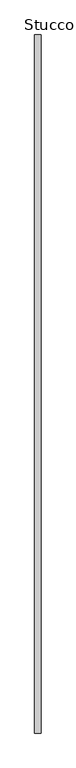
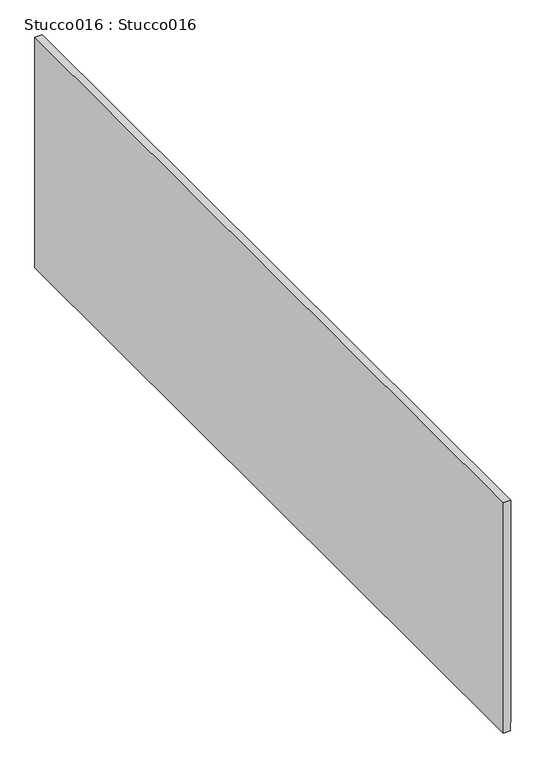
"""IFC4 building model written with IfcOpenShell, lengths in millimetres: proxy geometry, Stucco016 : Stucco016."""

import ifcopenshell
import ifcopenshell.guid

model = None  # the IFC model being written
_history = None  # IfcOwnerHistory: only IFC2X3 demands one
_inside = {}  # id of a spatial element -> (the spatial element, [elements in it])
_under = {}  # id of a project, library or spatial element -> (it, [spatial elements below it])
_declared = {}  # id of a project -> (the project, [libraries it declares])
_typed = {}  # id of a type object -> (the type object, [elements of that type])
_made_of = {}  # id of a material, layer set ... -> (it, [elements and type objects made of it])


def new_model(schema):
    """Start an empty IFC model of exactly this schema.

    Asked for "IFC4X3", IfcOpenShell would pick the latest addendum, in which some entities
    have other attributes; the version numbers below select the first issue.
    IFC2X3 requires an IfcOwnerHistory on every rooted entity: one is made here for all.
    """
    global model, _history
    if schema == "IFC4X3":
        model = ifcopenshell.file(schema_version=(4, 3, 0, 0))
    else:
        model = ifcopenshell.file(schema=schema)
    _inside.clear()
    _under.clear()
    _declared.clear()
    _typed.clear()
    _made_of.clear()
    _history = None
    if model.schema == "IFC2X3":
        org = make("IfcOrganization", Name="unknown")
        user = make(
            "IfcPersonAndOrganization",
            ThePerson=make("IfcPerson", FamilyName="unknown"),
            TheOrganization=org,
        )
        app = make(
            "IfcApplication",
            ApplicationDeveloper=org,
            Version="unknown",
            ApplicationFullName="unknown",
            ApplicationIdentifier="unknown",
        )
        _history = make(
            "IfcOwnerHistory",
            OwningUser=user,
            OwningApplication=app,
            ChangeAction="ADDED",
            CreationDate=0,
        )
    return model


def make(cls, **values):
    """One entity of the class cls with the attributes given. An attribute that is None is left unset."""
    return model.create_entity(
        cls, **{name: value for name, value in values.items() if value is not None}
    )


def rooted(cls, **values):
    """An entity with a GlobalId (a new one), such as an element, a storey or a relation."""
    return make(cls, GlobalId=ifcopenshell.guid.new(), OwnerHistory=_history, **values)


def si_unit(unit_type, name, prefix=None):
    """IfcSIUnit, for example si_unit("LENGTHUNIT", "METRE", prefix="MILLI")."""
    return make("IfcSIUnit", UnitType=unit_type, Prefix=prefix, Name=name)


def assignment(units):
    """IfcUnitAssignment: the units of a project."""
    return None if units is None else make("IfcUnitAssignment", Units=units)


def point(xyz):
    """IfcCartesianPoint."""
    return None if xyz is None else make("IfcCartesianPoint", Coordinates=xyz)


def direction(xyz):
    """IfcDirection."""
    return None if xyz is None else make("IfcDirection", DirectionRatios=xyz)


def frame(location, z_axis=None, x_axis=None):
    """IfcAxis2Placement3D, a coordinate frame: its origin and axes. An axis left out is left unset."""
    return make(
        "IfcAxis2Placement3D",
        Location=point(location),
        Axis=direction(z_axis),
        RefDirection=direction(x_axis),
    )


def origin():
    """The frame at (0, 0, 0) with its axes left unset."""
    return frame((0.0, 0.0, 0.0))


def place(relative_to, where):
    """IfcLocalPlacement: puts the frame where relative to a parent placement (None: the world)."""
    return make(
        "IfcLocalPlacement", PlacementRelTo=relative_to, RelativePlacement=where
    )


def context(
    kind, dimensions, precision=None, world=None, true_north=None, identifier=None
):
    """IfcGeometricRepresentationContext, for example the 3D "Model" context."""
    return make(
        "IfcGeometricRepresentationContext",
        ContextIdentifier=identifier,
        ContextType=kind,
        CoordinateSpaceDimension=dimensions,
        Precision=precision,
        WorldCoordinateSystem=world,
        TrueNorth=true_north,
    )


def project(units=None, contexts=None):
    """IfcProject with its units and contexts."""
    return rooted(
        "IfcProject",
        Name="project",
        RepresentationContexts=contexts,
        UnitsInContext=assignment(units),
    )


def spatial(cls, under=None, at=None, **own):
    """A site, building, storey or space (cls), placed at a placement, below another one or the project."""
    s = rooted(cls, ObjectPlacement=at, **own)
    if under is not None:
        _under.setdefault(under.id(), (under, []))[1].append(s)
    return s


def polyline(points):
    """IfcPolyline through the points."""
    return make("IfcPolyline", Points=[point(p) for p in points])


def outline(outer, holes=None, kind="AREA"):
    """IfcArbitraryClosedProfileDef: a profile drawn as a closed curve; with holes, ...WithVoids."""
    if holes is None:
        return make("IfcArbitraryClosedProfileDef", ProfileType=kind, OuterCurve=outer)
    return make(
        "IfcArbitraryProfileDefWithVoids",
        ProfileType=kind,
        OuterCurve=outer,
        InnerCurves=holes,
    )


def extrude(swept, where, along, depth):
    """IfcExtrudedAreaSolid: the profile swept, set in the frame where, extruded along a direction by depth."""
    return make(
        "IfcExtrudedAreaSolid",
        SweptArea=swept,
        Position=where,
        ExtrudedDirection=direction(along),
        Depth=depth,
    )


def shape(context_of_items, identifier, shape_type, items):
    """IfcShapeRepresentation: the items that make up one representation, for example the "Body"."""
    return make(
        "IfcShapeRepresentation",
        ContextOfItems=context_of_items,
        RepresentationIdentifier=identifier,
        RepresentationType=shape_type,
        Items=items,
    )


def source(mapping_origin, context_of_items, identifier, shape_type, items):
    """IfcRepresentationMap: a shape defined once, which mapped items show again and again."""
    return make(
        "IfcRepresentationMap",
        MappingOrigin=mapping_origin,
        MappedRepresentation=shape(context_of_items, identifier, shape_type, items),
    )


def transform(
    local_origin,
    x_axis=None,
    y_axis=None,
    z_axis=None,
    scale=None,
    scale2=None,
    scale3=None,
    uniform=True,
):
    """IfcCartesianTransformationOperator3D, or its non-uniform kind. x_axis, y_axis, z_axis: its Axis1, 2, 3."""
    if uniform:
        return make(
            "IfcCartesianTransformationOperator3D",
            Axis1=direction(x_axis),
            Axis2=direction(y_axis),
            LocalOrigin=point(local_origin),
            Scale=scale,
            Axis3=direction(z_axis),
        )
    return make(
        "IfcCartesianTransformationOperator3DnonUniform",
        Axis1=direction(x_axis),
        Axis2=direction(y_axis),
        LocalOrigin=point(local_origin),
        Scale=scale,
        Axis3=direction(z_axis),
        Scale2=scale2,
        Scale3=scale3,
    )


def mapped(mapping_source, mapping_target):
    """IfcMappedItem: shows the shape of a source again, moved by a transform."""
    return make(
        "IfcMappedItem", MappingSource=mapping_source, MappingTarget=mapping_target
    )


def made_of(thing, what):
    """Note that an element or type object is made of a material, layer set ...; save() writes the relation."""
    if what is not None:
        _made_of.setdefault(what.id(), (what, []))[1].append(thing)
    return thing


def element(
    cls,
    number,
    at=None,
    inside=None,
    cuts=None,
    type_object=None,
    material=None,
    context=None,
    identifier="Body",
    shape_type=None,
    held_by="IfcProductDefinitionShape",
    body=None,
    shapes=None,
    **own,
):
    """One element of the class cls, such as IfcWall. Its Tag is "e" and its number.

    at: its placement. inside: the storey or other place that contains it. cuts: it is an
    opening in that element (IfcRelVoidsElement). A single representation is given by context,
    identifier, shape_type and body (its items); several are given by shapes. held_by: the class
    of the entity that holds the representations. save() writes the other relations.
    """
    e = rooted(cls, Tag="e%d" % number, ObjectPlacement=at, **own)
    if body is not None:
        shapes = [shape(context, identifier, shape_type, body)]
    if shapes is not None:
        e.Representation = make(held_by, Representations=shapes)
    if inside is not None:
        _inside.setdefault(inside.id(), (inside, []))[1].append(e)
    if cuts is not None:
        rooted(
            "IfcRelVoidsElement", RelatingBuildingElement=cuts, RelatedOpeningElement=e
        )
    if type_object is not None:
        _typed.setdefault(type_object.id(), (type_object, []))[1].append(e)
    return made_of(e, material)


def aggregate(whole, parts):
    """IfcRelAggregates: a whole, such as a stair, and the parts it consists of."""
    return rooted("IfcRelAggregates", RelatingObject=whole, RelatedObjects=parts)


def save(model, path):
    """Write the relations noted so far, then the file.

    IfcRelAggregates (storeys below a building ...), IfcRelContainedInSpatialStructure (elements
    in a storey), IfcRelDefinesByType, IfcRelAssociatesMaterial and IfcRelDeclares: one each for
    every whole, place, type object, material and project.
    """
    for whole, parts in _under.values():
        aggregate(whole, parts)
    for where, things in _inside.values():
        rooted(
            "IfcRelContainedInSpatialStructure",
            RelatedElements=things,
            RelatingStructure=where,
        )
    for kind, things in _typed.values():
        rooted("IfcRelDefinesByType", RelatedObjects=things, RelatingType=kind)
    for what, things in _made_of.values():
        rooted("IfcRelAssociatesMaterial", RelatedObjects=things, RelatingMaterial=what)
    for by, libraries in _declared.values():
        rooted("IfcRelDeclares", RelatingContext=by, RelatedDefinitions=libraries)
    model.write(path)


def stucco016_stucco016_7183241d(model_context):
    return source(origin(), model_context, "Body", "SweptSolid", [
        extrude(outline(polyline([(39567.688258, -9269.4960354), (40145.4616445, -9269.4960354), (40145.4616445, -9287.27624), (39545.1576447, -9287.27624), (39545.1576447, -9270.7810557), (39567.688258, -9270.7810557), (39567.688258, -9269.4960354)])), frame((0.0, 7982.1530982, 0.0), z_axis=(0.0, 1.0, 0.0), x_axis=(0.0, 0.0, 1.0)), (0.0, 0.0, 1.0), 1999.9999999),
    ])


if __name__ == "__main__":
    model = new_model("IFC4")
    model_context = context("Model", 3, world=origin())
    ifc_project = project(units=[si_unit("LENGTHUNIT", "METRE", prefix="MILLI")], contexts=[model_context])
    site = spatial("IfcSite", under=ifc_project)
    building = spatial("IfcBuilding", under=site)
    placement = place(None, origin())
    stucco016_stucco016_shape = stucco016_stucco016_7183241d(model_context)
    element("IfcBuildingElementProxy", 1, Name="Stucco016 : Stucco016", ObjectType="Stucco016 : Stucco016", at=placement, inside=building, context=model_context, shape_type="MappedRepresentation", body=[
        mapped(stucco016_stucco016_shape, transform((0.0, 0.0, 0.0), x_axis=(1.0, 0.0, 0.0), y_axis=(0.0, 1.0, 0.0), z_axis=(0.0, 0.0, 1.0))),
    ])
    save(model, "model.ifc")

# Revit data of these elements
# Type "Stucco016 : Stucco016"
#   NameOverride = "Stucco016"
# Element 1 (IfcBuildingElementProxy, "Stucco016 : Stucco016")
#   Materials on its faces: "7/8\" SMOOTH TROWEL EXTERIOR STUCCO"
# Materials
#   "7/8\" SMOOTH TROWEL EXTERIOR STUCCO": class "Unassigned", colour RGB 255 255 255, transparency 0, Cost = 0
